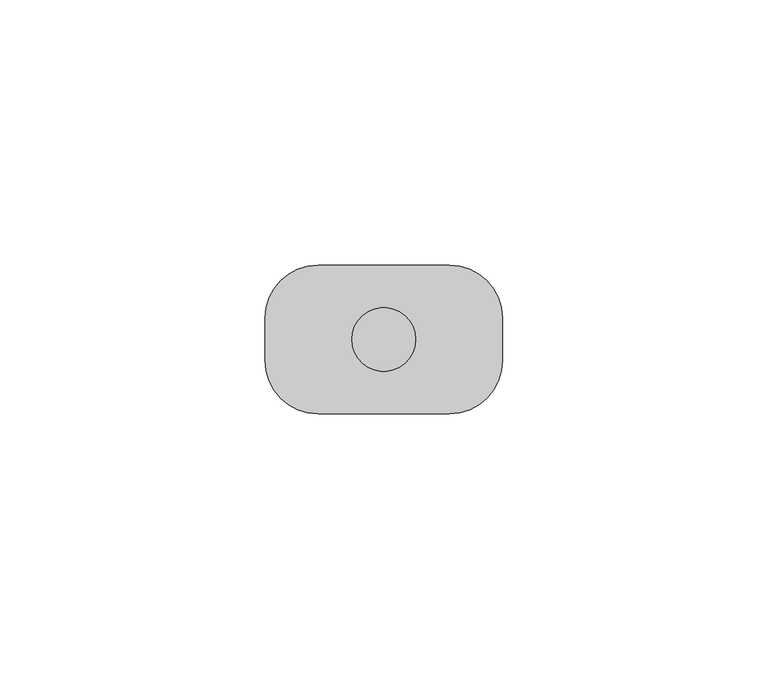
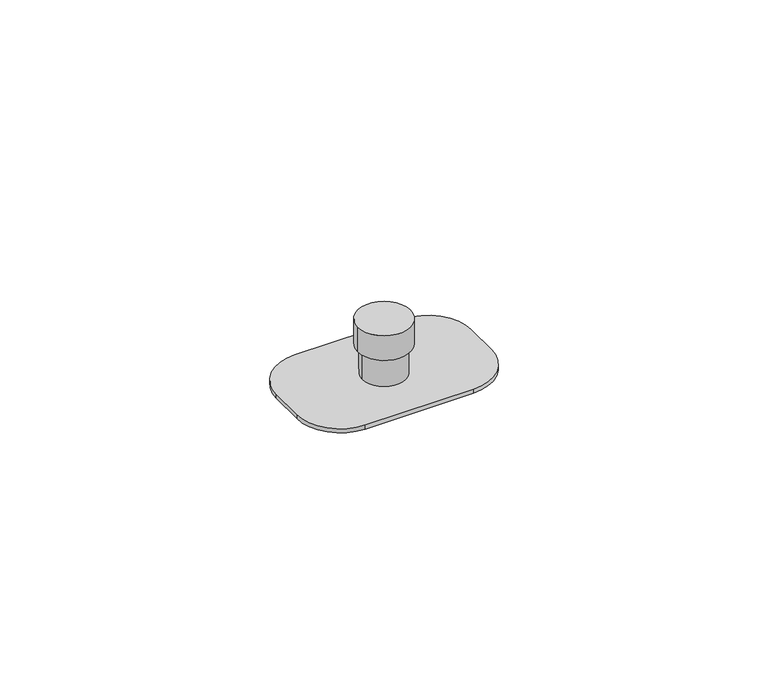
"""IFC4 building model written with IfcOpenShell, lengths in millimetres: proxy geometry, 12 mm Diameter Roller Wheel Sliding Wood Door Bottom Guide : 12 mm Diameter Roller Wheel Sliding Wood Door Bottom Guide."""

from ifc_helpers import new_model, si_unit, point, frame, frame_2d, origin, origin_with_axes, place, context, project, spatial, polyline, circle_curve, trimmed, segment, composite_curve, outline, extrude, source, transform, mapped, element, save


def generic_models_3738bab9(model_context):
    return source(origin(), model_context, "Body", "SweptSolid", [
        extrude(outline(composite_curve([segment(trimmed(circle_curve(frame_2d((0.0, -0.3941037)), 6.0151312), [point((-6.0151312, -0.3941037))], [point((6.0151312, -0.3941037))], False, "CARTESIAN"), True, "CONTINUOUS"), segment(trimmed(circle_curve(frame_2d((0.0, -0.3941037)), 6.0151312), [point((6.0151312, -0.3941037))], [point((-6.0151312, -0.3941037))], False, "CARTESIAN"), True, "CONTINUOUS")], self_intersect=False)), frame((0.0, 0.0, 8.0), z_axis=(0.0, 0.0, 1.0), x_axis=(1.0, 0.0, 0.0)), (0.0, 0.0, 1.0), 6.0),
        extrude(outline(composite_curve([segment(trimmed(circle_curve(frame_2d((0.0, -0.3941037)), 5.0), [point((-5.0, -0.3941037))], [point((5.0, -0.3941037))], False, "CARTESIAN"), True, "CONTINUOUS"), segment(trimmed(circle_curve(frame_2d((0.0, -0.3941037)), 5.0), [point((5.0, -0.3941037))], [point((-5.0, -0.3941037))], False, "CARTESIAN"), True, "CONTINUOUS")], self_intersect=False)), frame((0.0, 0.0, 1.0), z_axis=(0.0, 0.0, 1.0), x_axis=(1.0, 0.0, 0.0)), (0.0, 0.0, 1.0), 7.0),
        extrude(outline(composite_curve([segment(trimmed(circle_curve(frame_2d((12.4077768, 3.6058963)), 10.0), [point((12.4077768, 13.6058963))], [point((22.4077768, 3.6058963))], False, "CARTESIAN"), True, "CONTINUOUS"), segment(polyline([(22.4077768, 3.6058963), (22.4077768, -4.3941037)]), True, "CONTINUOUS"), segment(trimmed(circle_curve(frame_2d((12.4077768, -4.3941037)), 10.0), [point((22.4077768, -4.3941037))], [point((12.4077768, -14.3941037))], False, "CARTESIAN"), True, "CONTINUOUS"), segment(polyline([(12.4077768, -14.3941037), (-12.4077768, -14.3941037)]), True, "CONTINUOUS"), segment(trimmed(circle_curve(frame_2d((-12.4077768, -4.3941037)), 10.0), [point((-12.4077768, -14.3941037))], [point((-22.4077768, -4.3941037))], False, "CARTESIAN"), True, "CONTINUOUS"), segment(polyline([(-22.4077768, -4.3941037), (-22.4077768, 3.6058963)]), True, "CONTINUOUS"), segment(trimmed(circle_curve(frame_2d((-12.4077768, 3.6058963)), 10.0), [point((-22.4077768, 3.6058963))], [point((-12.4077768, 13.6058963))], False, "CARTESIAN"), True, "CONTINUOUS"), segment(polyline([(-12.4077768, 13.6058963), (12.4077768, 13.6058963)]), True, "CONTINUOUS")], self_intersect=False)), origin_with_axes(), (0.0, 0.0, 1.0), 1.0),
    ])


if __name__ == "__main__":
    model = new_model("IFC4")
    model_context = context("Model", 3, world=origin())
    ifc_project = project(units=[si_unit("LENGTHUNIT", "METRE", prefix="MILLI")], contexts=[model_context])
    site = spatial("IfcSite", under=ifc_project)
    building = spatial("IfcBuilding", under=site)
    placement = place(None, origin())
    generic_models_shape = generic_models_3738bab9(model_context)
    element("IfcBuildingElementProxy", 1, Name="12 mm Diameter Roller Wheel Sliding Wood Door Bottom Guide : 12 mm Diameter Roller Wheel Sliding Wood Door Bottom Guide", ObjectType="12 mm Diameter Roller Wheel Sliding Wood Door Bottom Guide : 12 mm Diameter Roller Wheel Sliding Wood Door Bottom Guide", at=placement, inside=building, context=model_context, shape_type="MappedRepresentation", body=[
        mapped(generic_models_shape, transform((0.0, 0.0, 0.0), x_axis=(1.0, 0.0, 0.0), y_axis=(0.0, 1.0, 0.0), z_axis=(0.0, 0.0, 1.0))),
    ])
    save(model, "model.ifc")

# Revit data of these elements
# Element 1 (IfcBuildingElementProxy, "12 mm Diameter Roller Wheel Sliding Wood Door Bottom Guide : 12 mm Diameter Roller Wheel Sliding Wood Door Bottom Guide")
#   Materials on its faces: "metal", "12 mm DIA. ROLLER WHEEL SLIDING WOOD DOOR BOTTOM GUIDE"
# Materials
#   "metal": class "Miscellaneous", colour RGB 127 127 127, transparency 0, Cost = 0
#   "12 mm DIA. ROLLER WHEEL SLIDING WOOD DOOR BOTTOM GUIDE": class "System", colour RGB 64 0 0, transparency 0, Cost = 0
